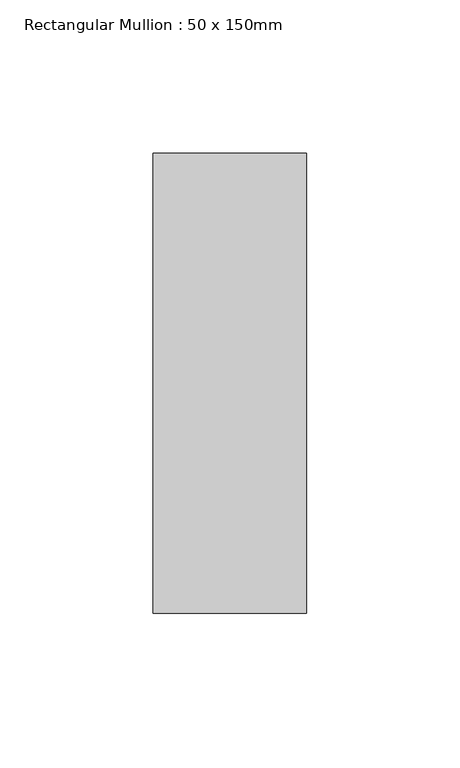
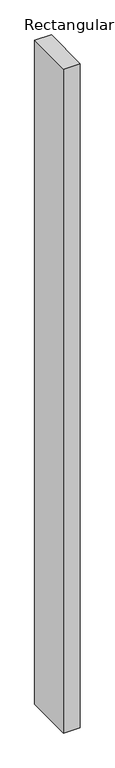
"""IFC4 building model written with IfcOpenShell, lengths in millimetres: member geometry, Rectangular Mullion : 50 x 150mm."""

from ifc_helpers import new_model, si_unit, frame, origin, place, context, project, spatial, polyline, outline, extrude, source, transform, mapped, element, save


def rectangular_mullion_50_x_150mm_bd4b94bd(model_context):
    return source(origin(), model_context, "Body", "SweptSolid", [
        extrude(outline(polyline([(0.0, 75.0), (0.0, -75.0), (-50.0, -75.0), (-50.0, 75.0), (0.0, 75.0)])), frame((0.0, 0.0, -2105.4462072), z_axis=(0.0, 0.0, 1.0), x_axis=(1.0, 0.0, 0.0)), (0.0, 0.0, 1.0), 2105.4462072),
    ])


if __name__ == "__main__":
    model = new_model("IFC4")
    model_context = context("Model", 3, world=origin())
    ifc_project = project(units=[si_unit("LENGTHUNIT", "METRE", prefix="MILLI")], contexts=[model_context])
    site = spatial("IfcSite", under=ifc_project)
    building = spatial("IfcBuilding", under=site)
    placement = place(None, origin())
    rectangular_mullion_50_x_150mm_shape = rectangular_mullion_50_x_150mm_bd4b94bd(model_context)
    element("IfcMember", 1, ObjectType="Rectangular Mullion : 50 x 150mm", at=placement, inside=building, context=model_context, shape_type="MappedRepresentation", body=[
        mapped(rectangular_mullion_50_x_150mm_shape, transform((0.0, 0.0, 0.0), x_axis=(1.0, 0.0, 0.0), y_axis=(0.0, 1.0, 0.0), z_axis=(0.0, 0.0, 1.0))),
    ])
    save(model, "model.ifc")

# Revit data of these elements
# Type "Rectangular Mullion : 50 x 150mm"
#   built-in parameter 1007304 = 0.492126 (stored number, unit not read)
#   built-in parameter 1007301 = 0.082021 (stored number, unit not read)
#   built-in parameter 1007300 = 0.082021 (stored number, unit not read)
# Element 1 (IfcMember, "Rectangular Mullion : 50 x 150mm")
#   Materials on its faces: "Aluminium"
# Materials
#   "Aluminium": class "Metal", colour RGB 247 247 247, transparency 0, Description = "Aluminium 6061", Cost = 0
